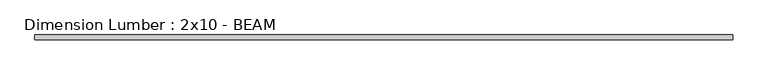
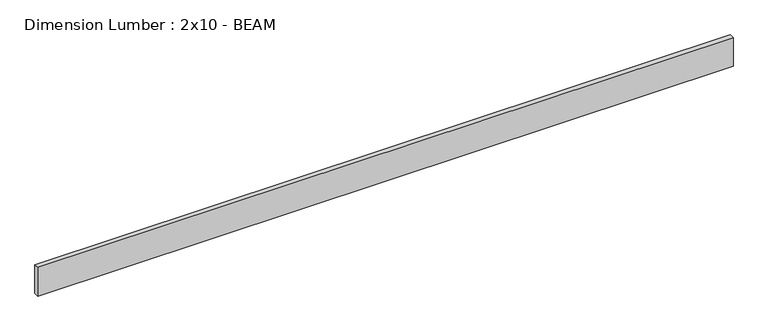
"""IFC4 building model written with IfcOpenShell, lengths in millimetres: beam geometry, Dimension Lumber : 2x10 - BEAM."""

import ifcopenshell
import ifcopenshell.guid

model = None  # the IFC model being written
_history = None  # IfcOwnerHistory: only IFC2X3 demands one
_inside = {}  # id of a spatial element -> (the spatial element, [elements in it])
_under = {}  # id of a project, library or spatial element -> (it, [spatial elements below it])
_declared = {}  # id of a project -> (the project, [libraries it declares])
_typed = {}  # id of a type object -> (the type object, [elements of that type])
_made_of = {}  # id of a material, layer set ... -> (it, [elements and type objects made of it])


def new_model(schema):
    """Start an empty IFC model of exactly this schema.

    Asked for "IFC4X3", IfcOpenShell would pick the latest addendum, in which some entities
    have other attributes; the version numbers below select the first issue.
    IFC2X3 requires an IfcOwnerHistory on every rooted entity: one is made here for all.
    """
    global model, _history
    if schema == "IFC4X3":
        model = ifcopenshell.file(schema_version=(4, 3, 0, 0))
    else:
        model = ifcopenshell.file(schema=schema)
    _inside.clear()
    _under.clear()
    _declared.clear()
    _typed.clear()
    _made_of.clear()
    _history = None
    if model.schema == "IFC2X3":
        org = make("IfcOrganization", Name="unknown")
        user = make(
            "IfcPersonAndOrganization",
            ThePerson=make("IfcPerson", FamilyName="unknown"),
            TheOrganization=org,
        )
        app = make(
            "IfcApplication",
            ApplicationDeveloper=org,
            Version="unknown",
            ApplicationFullName="unknown",
            ApplicationIdentifier="unknown",
        )
        _history = make(
            "IfcOwnerHistory",
            OwningUser=user,
            OwningApplication=app,
            ChangeAction="ADDED",
            CreationDate=0,
        )
    return model


def make(cls, **values):
    """One entity of the class cls with the attributes given. An attribute that is None is left unset."""
    return model.create_entity(
        cls, **{name: value for name, value in values.items() if value is not None}
    )


def rooted(cls, **values):
    """An entity with a GlobalId (a new one), such as an element, a storey or a relation."""
    return make(cls, GlobalId=ifcopenshell.guid.new(), OwnerHistory=_history, **values)


def si_unit(unit_type, name, prefix=None):
    """IfcSIUnit, for example si_unit("LENGTHUNIT", "METRE", prefix="MILLI")."""
    return make("IfcSIUnit", UnitType=unit_type, Prefix=prefix, Name=name)


def assignment(units):
    """IfcUnitAssignment: the units of a project."""
    return None if units is None else make("IfcUnitAssignment", Units=units)


def point(xyz):
    """IfcCartesianPoint."""
    return None if xyz is None else make("IfcCartesianPoint", Coordinates=xyz)


def direction(xyz):
    """IfcDirection."""
    return None if xyz is None else make("IfcDirection", DirectionRatios=xyz)


def frame(location, z_axis=None, x_axis=None):
    """IfcAxis2Placement3D, a coordinate frame: its origin and axes. An axis left out is left unset."""
    return make(
        "IfcAxis2Placement3D",
        Location=point(location),
        Axis=direction(z_axis),
        RefDirection=direction(x_axis),
    )


def origin():
    """The frame at (0, 0, 0) with its axes left unset."""
    return frame((0.0, 0.0, 0.0))


def place(relative_to, where):
    """IfcLocalPlacement: puts the frame where relative to a parent placement (None: the world)."""
    return make(
        "IfcLocalPlacement", PlacementRelTo=relative_to, RelativePlacement=where
    )


def context(
    kind, dimensions, precision=None, world=None, true_north=None, identifier=None
):
    """IfcGeometricRepresentationContext, for example the 3D "Model" context."""
    return make(
        "IfcGeometricRepresentationContext",
        ContextIdentifier=identifier,
        ContextType=kind,
        CoordinateSpaceDimension=dimensions,
        Precision=precision,
        WorldCoordinateSystem=world,
        TrueNorth=true_north,
    )


def project(units=None, contexts=None):
    """IfcProject with its units and contexts."""
    return rooted(
        "IfcProject",
        Name="project",
        RepresentationContexts=contexts,
        UnitsInContext=assignment(units),
    )


def spatial(cls, under=None, at=None, **own):
    """A site, building, storey or space (cls), placed at a placement, below another one or the project."""
    s = rooted(cls, ObjectPlacement=at, **own)
    if under is not None:
        _under.setdefault(under.id(), (under, []))[1].append(s)
    return s


def polyline(points):
    """IfcPolyline through the points."""
    return make("IfcPolyline", Points=[point(p) for p in points])


def outline(outer, holes=None, kind="AREA"):
    """IfcArbitraryClosedProfileDef: a profile drawn as a closed curve; with holes, ...WithVoids."""
    if holes is None:
        return make("IfcArbitraryClosedProfileDef", ProfileType=kind, OuterCurve=outer)
    return make(
        "IfcArbitraryProfileDefWithVoids",
        ProfileType=kind,
        OuterCurve=outer,
        InnerCurves=holes,
    )


def extrude(swept, where, along, depth):
    """IfcExtrudedAreaSolid: the profile swept, set in the frame where, extruded along a direction by depth."""
    return make(
        "IfcExtrudedAreaSolid",
        SweptArea=swept,
        Position=where,
        ExtrudedDirection=direction(along),
        Depth=depth,
    )


def shape(context_of_items, identifier, shape_type, items):
    """IfcShapeRepresentation: the items that make up one representation, for example the "Body"."""
    return make(
        "IfcShapeRepresentation",
        ContextOfItems=context_of_items,
        RepresentationIdentifier=identifier,
        RepresentationType=shape_type,
        Items=items,
    )


def source(mapping_origin, context_of_items, identifier, shape_type, items):
    """IfcRepresentationMap: a shape defined once, which mapped items show again and again."""
    return make(
        "IfcRepresentationMap",
        MappingOrigin=mapping_origin,
        MappedRepresentation=shape(context_of_items, identifier, shape_type, items),
    )


def transform(
    local_origin,
    x_axis=None,
    y_axis=None,
    z_axis=None,
    scale=None,
    scale2=None,
    scale3=None,
    uniform=True,
):
    """IfcCartesianTransformationOperator3D, or its non-uniform kind. x_axis, y_axis, z_axis: its Axis1, 2, 3."""
    if uniform:
        return make(
            "IfcCartesianTransformationOperator3D",
            Axis1=direction(x_axis),
            Axis2=direction(y_axis),
            LocalOrigin=point(local_origin),
            Scale=scale,
            Axis3=direction(z_axis),
        )
    return make(
        "IfcCartesianTransformationOperator3DnonUniform",
        Axis1=direction(x_axis),
        Axis2=direction(y_axis),
        LocalOrigin=point(local_origin),
        Scale=scale,
        Axis3=direction(z_axis),
        Scale2=scale2,
        Scale3=scale3,
    )


def mapped(mapping_source, mapping_target):
    """IfcMappedItem: shows the shape of a source again, moved by a transform."""
    return make(
        "IfcMappedItem", MappingSource=mapping_source, MappingTarget=mapping_target
    )


def made_of(thing, what):
    """Note that an element or type object is made of a material, layer set ...; save() writes the relation."""
    if what is not None:
        _made_of.setdefault(what.id(), (what, []))[1].append(thing)
    return thing


def element(
    cls,
    number,
    at=None,
    inside=None,
    cuts=None,
    type_object=None,
    material=None,
    context=None,
    identifier="Body",
    shape_type=None,
    held_by="IfcProductDefinitionShape",
    body=None,
    shapes=None,
    **own,
):
    """One element of the class cls, such as IfcWall. Its Tag is "e" and its number.

    at: its placement. inside: the storey or other place that contains it. cuts: it is an
    opening in that element (IfcRelVoidsElement). A single representation is given by context,
    identifier, shape_type and body (its items); several are given by shapes. held_by: the class
    of the entity that holds the representations. save() writes the other relations.
    """
    e = rooted(cls, Tag="e%d" % number, ObjectPlacement=at, **own)
    if body is not None:
        shapes = [shape(context, identifier, shape_type, body)]
    if shapes is not None:
        e.Representation = make(held_by, Representations=shapes)
    if inside is not None:
        _inside.setdefault(inside.id(), (inside, []))[1].append(e)
    if cuts is not None:
        rooted(
            "IfcRelVoidsElement", RelatingBuildingElement=cuts, RelatedOpeningElement=e
        )
    if type_object is not None:
        _typed.setdefault(type_object.id(), (type_object, []))[1].append(e)
    return made_of(e, material)


def aggregate(whole, parts):
    """IfcRelAggregates: a whole, such as a stair, and the parts it consists of."""
    return rooted("IfcRelAggregates", RelatingObject=whole, RelatedObjects=parts)


def save(model, path):
    """Write the relations noted so far, then the file.

    IfcRelAggregates (storeys below a building ...), IfcRelContainedInSpatialStructure (elements
    in a storey), IfcRelDefinesByType, IfcRelAssociatesMaterial and IfcRelDeclares: one each for
    every whole, place, type object, material and project.
    """
    for whole, parts in _under.values():
        aggregate(whole, parts)
    for where, things in _inside.values():
        rooted(
            "IfcRelContainedInSpatialStructure",
            RelatedElements=things,
            RelatingStructure=where,
        )
    for kind, things in _typed.values():
        rooted("IfcRelDefinesByType", RelatedObjects=things, RelatingType=kind)
    for what, things in _made_of.values():
        rooted("IfcRelAssociatesMaterial", RelatedObjects=things, RelatingMaterial=what)
    for by, libraries in _declared.values():
        rooted("IfcRelDeclares", RelatingContext=by, RelatedDefinitions=libraries)
    model.write(path)


def dimension_lumber_2x10_beam_93704977(model_context):
    return source(origin(), model_context, "Body", "SweptSolid", [
        extrude(outline(polyline([(2714.2903727, 19.05), (2714.2903727, -19.05), (-2695.2403727, -19.05), (-2695.2403727, 19.05), (2714.2903727, 19.05)])), frame((0.0, 0.0, -117.475), z_axis=(0.0, 0.0, 1.0), x_axis=(1.0, 0.0, 0.0)), (0.0, 0.0, 1.0), 234.95),
    ])


if __name__ == "__main__":
    model = new_model("IFC4")
    model_context = context("Model", 3, world=origin())
    ifc_project = project(units=[si_unit("LENGTHUNIT", "METRE", prefix="MILLI")], contexts=[model_context])
    site = spatial("IfcSite", under=ifc_project)
    building = spatial("IfcBuilding", under=site)
    placement = place(None, origin())
    dimension_lumber_2x10_beam_shape = dimension_lumber_2x10_beam_93704977(model_context)
    element("IfcBeam", 1, ObjectType="Dimension Lumber : 2x10 - BEAM", at=placement, inside=building, context=model_context, shape_type="MappedRepresentation", body=[
        mapped(dimension_lumber_2x10_beam_shape, transform((0.0, 0.0, 0.0), x_axis=(1.0, 0.0, 0.0), y_axis=(0.0, 1.0, 0.0), z_axis=(0.0, 0.0, 1.0))),
    ])
    save(model, "model.ifc")

# Revit data of these elements
# Type "Dimension Lumber : 2x10 - BEAM"
#   Assembly Code = "B10"
#   A = 0.0755556 SF
#   Length [instance default] = 5' - 0"
#   b = 0' - 1 1/2"
#   d = 0' - 9 1/4"
#   Structural Material = (3) SISTERED 2X10s AT BEAM
# Element 1 (IfcBeam, "Dimension Lumber : 2x10 - BEAM")
#   Materials on its faces: "(3) SISTERED 2X10s AT BEAM"
# Materials
#   "(3) SISTERED 2X10s AT BEAM": class "Wood", colour RGB 234 198 147, transparency 0, Description = "Pinus Echinata", Cost = 0
